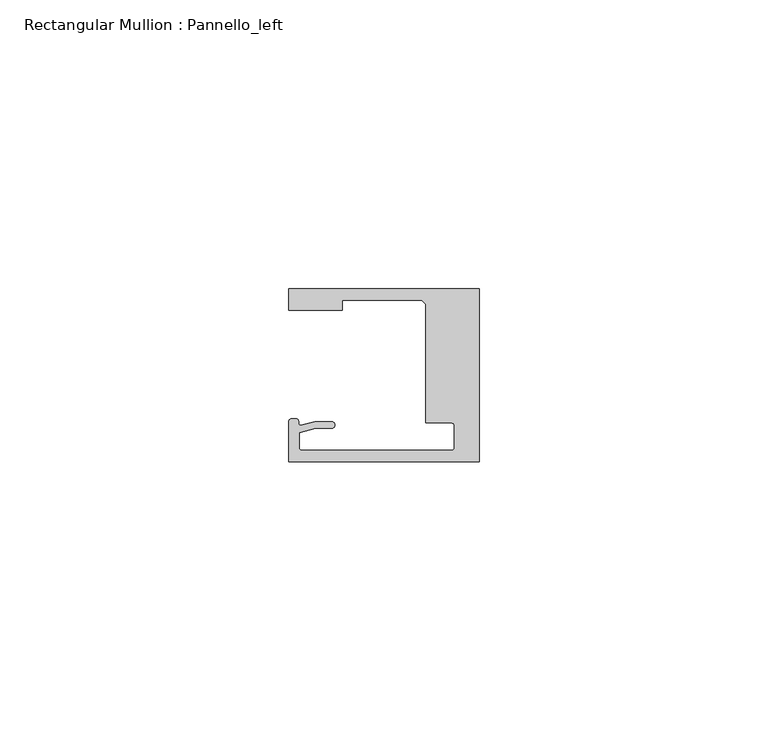
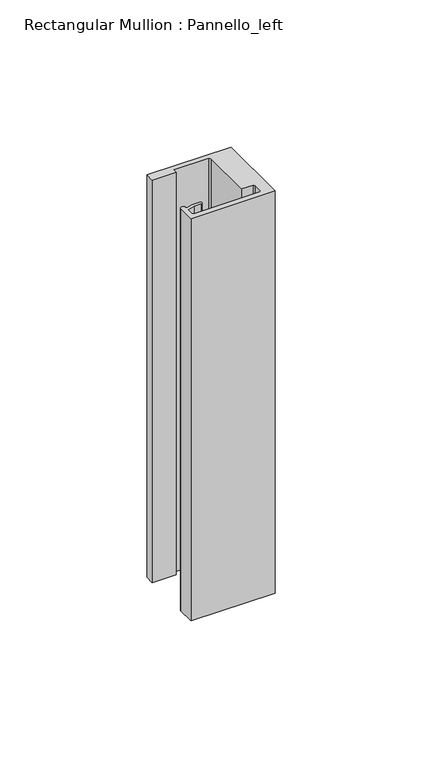
"""IFC4 building model written with IfcOpenShell, lengths in millimetres: member geometry, Rectangular Mullion : Pannello_left."""

import ifcopenshell
import ifcopenshell.guid

model = None  # the IFC model being written
_history = None  # IfcOwnerHistory: only IFC2X3 demands one
_inside = {}  # id of a spatial element -> (the spatial element, [elements in it])
_under = {}  # id of a project, library or spatial element -> (it, [spatial elements below it])
_declared = {}  # id of a project -> (the project, [libraries it declares])
_typed = {}  # id of a type object -> (the type object, [elements of that type])
_made_of = {}  # id of a material, layer set ... -> (it, [elements and type objects made of it])


def new_model(schema):
    """Start an empty IFC model of exactly this schema.

    Asked for "IFC4X3", IfcOpenShell would pick the latest addendum, in which some entities
    have other attributes; the version numbers below select the first issue.
    IFC2X3 requires an IfcOwnerHistory on every rooted entity: one is made here for all.
    """
    global model, _history
    if schema == "IFC4X3":
        model = ifcopenshell.file(schema_version=(4, 3, 0, 0))
    else:
        model = ifcopenshell.file(schema=schema)
    _inside.clear()
    _under.clear()
    _declared.clear()
    _typed.clear()
    _made_of.clear()
    _history = None
    if model.schema == "IFC2X3":
        org = make("IfcOrganization", Name="unknown")
        user = make(
            "IfcPersonAndOrganization",
            ThePerson=make("IfcPerson", FamilyName="unknown"),
            TheOrganization=org,
        )
        app = make(
            "IfcApplication",
            ApplicationDeveloper=org,
            Version="unknown",
            ApplicationFullName="unknown",
            ApplicationIdentifier="unknown",
        )
        _history = make(
            "IfcOwnerHistory",
            OwningUser=user,
            OwningApplication=app,
            ChangeAction="ADDED",
            CreationDate=0,
        )
    return model


def make(cls, **values):
    """One entity of the class cls with the attributes given. An attribute that is None is left unset."""
    return model.create_entity(
        cls, **{name: value for name, value in values.items() if value is not None}
    )


def rooted(cls, **values):
    """An entity with a GlobalId (a new one), such as an element, a storey or a relation."""
    return make(cls, GlobalId=ifcopenshell.guid.new(), OwnerHistory=_history, **values)


def si_unit(unit_type, name, prefix=None):
    """IfcSIUnit, for example si_unit("LENGTHUNIT", "METRE", prefix="MILLI")."""
    return make("IfcSIUnit", UnitType=unit_type, Prefix=prefix, Name=name)


def assignment(units):
    """IfcUnitAssignment: the units of a project."""
    return None if units is None else make("IfcUnitAssignment", Units=units)


def point(xyz):
    """IfcCartesianPoint."""
    return None if xyz is None else make("IfcCartesianPoint", Coordinates=xyz)


def direction(xyz):
    """IfcDirection."""
    return None if xyz is None else make("IfcDirection", DirectionRatios=xyz)


def frame(location, z_axis=None, x_axis=None):
    """IfcAxis2Placement3D, a coordinate frame: its origin and axes. An axis left out is left unset."""
    return make(
        "IfcAxis2Placement3D",
        Location=point(location),
        Axis=direction(z_axis),
        RefDirection=direction(x_axis),
    )


def origin():
    """The frame at (0, 0, 0) with its axes left unset."""
    return frame((0.0, 0.0, 0.0))


def place(relative_to, where):
    """IfcLocalPlacement: puts the frame where relative to a parent placement (None: the world)."""
    return make(
        "IfcLocalPlacement", PlacementRelTo=relative_to, RelativePlacement=where
    )


def context(
    kind, dimensions, precision=None, world=None, true_north=None, identifier=None
):
    """IfcGeometricRepresentationContext, for example the 3D "Model" context."""
    return make(
        "IfcGeometricRepresentationContext",
        ContextIdentifier=identifier,
        ContextType=kind,
        CoordinateSpaceDimension=dimensions,
        Precision=precision,
        WorldCoordinateSystem=world,
        TrueNorth=true_north,
    )


def project(units=None, contexts=None):
    """IfcProject with its units and contexts."""
    return rooted(
        "IfcProject",
        Name="project",
        RepresentationContexts=contexts,
        UnitsInContext=assignment(units),
    )


def spatial(cls, under=None, at=None, **own):
    """A site, building, storey or space (cls), placed at a placement, below another one or the project."""
    s = rooted(cls, ObjectPlacement=at, **own)
    if under is not None:
        _under.setdefault(under.id(), (under, []))[1].append(s)
    return s


def polyline(points):
    """IfcPolyline through the points."""
    return make("IfcPolyline", Points=[point(p) for p in points])


def circle_curve(where, radius):
    """IfcCircle in the frame where."""
    return make("IfcCircle", Position=where, Radius=radius)


def shape(context_of_items, identifier, shape_type, items):
    """IfcShapeRepresentation: the items that make up one representation, for example the "Body"."""
    return make(
        "IfcShapeRepresentation",
        ContextOfItems=context_of_items,
        RepresentationIdentifier=identifier,
        RepresentationType=shape_type,
        Items=items,
    )


def source(mapping_origin, context_of_items, identifier, shape_type, items):
    """IfcRepresentationMap: a shape defined once, which mapped items show again and again."""
    return make(
        "IfcRepresentationMap",
        MappingOrigin=mapping_origin,
        MappedRepresentation=shape(context_of_items, identifier, shape_type, items),
    )


def transform(
    local_origin,
    x_axis=None,
    y_axis=None,
    z_axis=None,
    scale=None,
    scale2=None,
    scale3=None,
    uniform=True,
):
    """IfcCartesianTransformationOperator3D, or its non-uniform kind. x_axis, y_axis, z_axis: its Axis1, 2, 3."""
    if uniform:
        return make(
            "IfcCartesianTransformationOperator3D",
            Axis1=direction(x_axis),
            Axis2=direction(y_axis),
            LocalOrigin=point(local_origin),
            Scale=scale,
            Axis3=direction(z_axis),
        )
    return make(
        "IfcCartesianTransformationOperator3DnonUniform",
        Axis1=direction(x_axis),
        Axis2=direction(y_axis),
        LocalOrigin=point(local_origin),
        Scale=scale,
        Axis3=direction(z_axis),
        Scale2=scale2,
        Scale3=scale3,
    )


def mapped(mapping_source, mapping_target):
    """IfcMappedItem: shows the shape of a source again, moved by a transform."""
    return make(
        "IfcMappedItem", MappingSource=mapping_source, MappingTarget=mapping_target
    )


def made_of(thing, what):
    """Note that an element or type object is made of a material, layer set ...; save() writes the relation."""
    if what is not None:
        _made_of.setdefault(what.id(), (what, []))[1].append(thing)
    return thing


def element(
    cls,
    number,
    at=None,
    inside=None,
    cuts=None,
    type_object=None,
    material=None,
    context=None,
    identifier="Body",
    shape_type=None,
    held_by="IfcProductDefinitionShape",
    body=None,
    shapes=None,
    **own,
):
    """One element of the class cls, such as IfcWall. Its Tag is "e" and its number.

    at: its placement. inside: the storey or other place that contains it. cuts: it is an
    opening in that element (IfcRelVoidsElement). A single representation is given by context,
    identifier, shape_type and body (its items); several are given by shapes. held_by: the class
    of the entity that holds the representations. save() writes the other relations.
    """
    e = rooted(cls, Tag="e%d" % number, ObjectPlacement=at, **own)
    if body is not None:
        shapes = [shape(context, identifier, shape_type, body)]
    if shapes is not None:
        e.Representation = make(held_by, Representations=shapes)
    if inside is not None:
        _inside.setdefault(inside.id(), (inside, []))[1].append(e)
    if cuts is not None:
        rooted(
            "IfcRelVoidsElement", RelatingBuildingElement=cuts, RelatedOpeningElement=e
        )
    if type_object is not None:
        _typed.setdefault(type_object.id(), (type_object, []))[1].append(e)
    return made_of(e, material)


def aggregate(whole, parts):
    """IfcRelAggregates: a whole, such as a stair, and the parts it consists of."""
    return rooted("IfcRelAggregates", RelatingObject=whole, RelatedObjects=parts)


def save(model, path):
    """Write the relations noted so far, then the file.

    IfcRelAggregates (storeys below a building ...), IfcRelContainedInSpatialStructure (elements
    in a storey), IfcRelDefinesByType, IfcRelAssociatesMaterial and IfcRelDeclares: one each for
    every whole, place, type object, material and project.
    """
    for whole, parts in _under.values():
        aggregate(whole, parts)
    for where, things in _inside.values():
        rooted(
            "IfcRelContainedInSpatialStructure",
            RelatedElements=things,
            RelatingStructure=where,
        )
    for kind, things in _typed.values():
        rooted("IfcRelDefinesByType", RelatedObjects=things, RelatingType=kind)
    for what, things in _made_of.values():
        rooted("IfcRelAssociatesMaterial", RelatedObjects=things, RelatingMaterial=what)
    for by, libraries in _declared.values():
        rooted("IfcRelDeclares", RelatingContext=by, RelatedDefinitions=libraries)
    model.write(path)


def plane_surface(at):
    """IfcPlane: the flat surface through the origin of the frame at, square to its z axis."""
    return make("IfcPlane", Position=at)


def cylinder_surface(at, radius):
    """IfcCylindricalSurface: all points at the distance radius from the z axis of the frame at."""
    return make("IfcCylindricalSurface", Position=at, Radius=radius)


def revolved_surface(curve, axis_point, axis_direction):
    """IfcSurfaceOfRevolution: the curve turned about the line through axis_point along axis_direction."""
    return make(
        "IfcSurfaceOfRevolution",
        SweptCurve=make("IfcArbitraryOpenProfileDef", ProfileType="CURVE", Curve=curve),
        AxisPosition=make("IfcAxis1Placement", Location=point(axis_point), Axis=direction(axis_direction)),
    )


def extruded_surface(curve, direction_of_extrusion, depth):
    """IfcSurfaceOfLinearExtrusion: the curve pushed along a direction by depth."""
    return make(
        "IfcSurfaceOfLinearExtrusion",
        SweptCurve=make("IfcArbitraryOpenProfileDef", ProfileType="CURVE", Curve=curve),
        ExtrudedDirection=direction(direction_of_extrusion),
        Depth=depth,
    )


def spline_curve(degree, points, multiplicities, knots, weights=None):
    """IfcBSplineCurveWithKnots; with weights, IfcRationalBSplineCurveWithKnots."""
    own = dict(
        Degree=degree,
        ControlPointsList=[point(p) for p in points],
        CurveForm="UNSPECIFIED",
        ClosedCurve=False,
        SelfIntersect=False,
        KnotMultiplicities=multiplicities,
        Knots=knots,
        KnotSpec="UNSPECIFIED",
    )
    if weights is None:
        return make("IfcBSplineCurveWithKnots", **own)
    return make("IfcRationalBSplineCurveWithKnots", WeightsData=weights, **own)


def advanced_brep(points, edges, surfaces, faces):
    """IfcAdvancedBrep: a solid bounded by faces that lie on surfaces and meet in shared edges.

    An edge is (start, end): straight between two places in points (the first is 0);
    or (start, end, curve); or (start, end, curve, False) where it runs against its curve.
    A face is (place in surfaces, loops), or (place, loops, False) where it looks against
    its surface's normal. A loop lists edges by number (the first is 1), with a minus sign
    where the edge is run from its end to its start. The first loop is the outer one.
    """
    corners = [point(p) for p in points]
    vertices = [make("IfcVertexPoint", VertexGeometry=c) for c in corners]
    made = []
    for start, end, *more in edges:
        made.append(
            make(
                "IfcEdgeCurve",
                EdgeStart=vertices[start],
                EdgeEnd=vertices[end],
                EdgeGeometry=more[0] if more else make("IfcPolyline", Points=[corners[start], corners[end]]),
                SameSense=more[1] if len(more) > 1 else True,
            )
        )
    hull = []
    for where, loops, *sense in faces:
        bounds = []
        for j, loop in enumerate(loops):
            ring = [make("IfcOrientedEdge", EdgeElement=made[abs(k) - 1], Orientation=k > 0) for k in loop]
            bounds.append(
                make(
                    "IfcFaceOuterBound" if j == 0 else "IfcFaceBound",
                    Bound=make("IfcEdgeLoop", EdgeList=ring),
                    Orientation=True,
                )
            )
        hull.append(make("IfcAdvancedFace", Bounds=bounds, FaceSurface=surfaces[where], SameSense=sense[0] if sense else True))
    return make("IfcAdvancedBrep", Outer=make("IfcClosedShell", CfsFaces=hull))


def rectangular_mullion_pannello_left_9b2e0e1e(model_context):
    return source(origin(), model_context, "Body", "AdvancedBrep", [
        advanced_brep(
        [(-33.0, 15.0, 0.0), (-33.0, 11.3000004, 0.0), (-23.700041, 11.3000004, 0.0), (-23.700041, 13.0000004, 0.0), (-10.0000103, 13.0000004, 0.0), (-9.2999726, 12.2999849, 0.0), (-9.2999726, -8.2500595, 0.0), (-4.7999726, -8.2500595, 0.0), (-4.2999726, -8.7500595, 0.0), (-4.2999726, -12.50001, 0.0), (-4.7999726, -13.00001, 0.0), (-30.69998, -13.00001, 0.0), (-31.19998, -12.50001, 0.0), (-31.19998, -9.9657591, 0.0), (-28.3419477, -9.1999523, 0.0), (-25.59998, -9.1999523, 0.0), (-25.59998, -7.9999523, 0.0), (-28.4999305, -7.9999523, 0.0), (-30.9223017, -8.6490241, 0.0), (-33.0000135, -8.0000472, 0.0), (-33.0000135, -15.0, 0.0), (0.0, -15.0, 0.0), (0.0, 15.0, 0.0), (-33.0, 15.0, -166.9999865), (0.0, 15.0, -166.9999865), (0.0, -15.0, -166.9999865), (-33.0000135, -15.0, -166.9999865), (-33.0000135, -8.0000472, -166.9999865), (-30.9223017, -8.6490241, -166.9999865), (-28.4999305, -7.9999523, -166.9999865), (-25.59998, -7.9999523, -166.9999865), (-25.59998, -9.1999523, -166.9999865), (-28.3419477, -9.1999523, -166.9999865), (-31.19998, -9.9657591, -166.9999865), (-31.19998, -12.50001, -166.9999865), (-30.69998, -13.00001, -166.9999865), (-4.7999726, -13.00001, -166.9999865), (-4.2999726, -12.50001, -166.9999865), (-4.2999726, -8.7500595, -166.9999865), (-4.7999726, -8.2500595, -166.9999865), (-9.2999726, -8.2500595, -166.9999865), (-9.2999726, 12.2999849, -166.9999865), (-10.0000103, 13.0000004, -166.9999865), (-23.700041, 13.0000004, -166.9999865), (-23.700041, 11.3000004, -166.9999865), (-33.0, 11.3000004, -166.9999865)],
        [
            (0, 1),
            (1, 2),
            (2, 3),
            (3, 4),
            (4, 5),
            (5, 6),
            (6, 7),
            (7, 8, circle_curve(frame((-4.7999726, -8.7500595, 0.0), z_axis=(0.0, 0.0, -1.0), x_axis=(0.0, 1.0, 0.0)), 0.5)),
            (8, 9),
            (9, 10, circle_curve(frame((-4.7999726, -12.50001, 0.0), z_axis=(0.0, 0.0, -1.0), x_axis=(1.0, 0.0, 0.0)), 0.5)),
            (10, 11),
            (11, 12, circle_curve(frame((-30.69998, -12.50001, 0.0), z_axis=(0.0, 0.0, -1.0), x_axis=(0.0, -1.0, 0.0)), 0.5)),
            (12, 13),
            (13, 14),
            (14, 15),
            (15, 16, circle_curve(frame((-25.59998, -8.5999523, 0.0), z_axis=(0.0, 0.0, 1.0), x_axis=(0.0, -1.0, 0.0)), 0.6)),
            (16, 17),
            (17, 18),
            (18, 19, spline_curve(3, [(-30.9223017, -8.6490241, 0.0), (-31.312054066, -8.717747958, 0.0), (-31.298563602, -8.366228555, 0.0), (-31.305645054, -7.690065204, 0.0), (-31.357433266, -7.563996614, 0.0), (-32.262327879, -7.456527435, 0.0), (-33.0000135, -7.457047519, 0.0), (-33.0000135, -8.0000472, 0.0)], [4, 2, 2, 4], [0.0, 0.001840817752199412, 0.004996616814974408, 0.007702013405570312])),
            (19, 20),
            (20, 21),
            (21, 22),
            (22, 0),
            (23, 24),
            (24, 25),
            (25, 26),
            (26, 27),
            (27, 28, spline_curve(3, [(-33.0000135, -8.0000472, -166.9999865), (-33.0000135, -7.457047519, -166.9999865), (-32.262327879, -7.456527435, -166.9999865), (-31.357433266, -7.563996614, -166.9999865), (-31.305645054, -7.690065204, -166.9999865), (-31.298563602, -8.366228555, -166.9999865), (-31.312054066, -8.717747958, -166.9999865), (-30.9223017, -8.6490241, -166.9999865)], [4, 2, 2, 4], [0.0, 0.0027053965905959043, 0.0058611956533709, 0.007702013405570312])),
            (28, 29),
            (29, 30),
            (30, 31, circle_curve(frame((-25.59998, -8.5999523, -166.9999865), z_axis=(0.0, 0.0, -1.0), x_axis=(0.0, -1.0, 0.0)), 0.6)),
            (31, 32),
            (32, 33),
            (33, 34),
            (34, 35, circle_curve(frame((-30.69998, -12.50001, -166.9999865), z_axis=(0.0, 0.0, 1.0), x_axis=(0.0, -1.0, 0.0)), 0.5)),
            (35, 36),
            (36, 37, circle_curve(frame((-4.7999726, -12.50001, -166.9999865), z_axis=(0.0, 0.0, 1.0), x_axis=(1.0, 0.0, 0.0)), 0.5)),
            (37, 38),
            (38, 39, circle_curve(frame((-4.7999726, -8.7500595, -166.9999865), z_axis=(0.0, 0.0, 1.0), x_axis=(0.0, 1.0, 0.0)), 0.5)),
            (39, 40),
            (40, 41),
            (41, 42),
            (42, 43),
            (43, 44),
            (44, 45),
            (45, 23),
            (0, 23),
            (45, 1),
            (44, 2),
            (43, 3),
            (42, 4),
            (41, 5),
            (40, 6),
            (39, 7),
            (38, 8),
            (37, 9),
            (36, 10),
            (35, 11),
            (34, 12),
            (33, 13),
            (32, 14),
            (31, 15),
            (30, 16),
            (29, 17),
            (28, 18),
            (27, 19),
            (26, 20),
            (25, 21),
            (24, 22),
        ],
        [
            plane_surface(frame((0.0, -36.2491502, 0.0), z_axis=(0.0, 0.0, 1.0), x_axis=(-1.0, 0.0, 0.0))),
            plane_surface(frame((0.0, -36.2491502, -166.9999865), z_axis=(0.0, 0.0, -1.0), x_axis=(-1.0, 0.0, 0.0))),
            plane_surface(frame((-33.0, 15.0, 0.0), z_axis=(-1.0, 0.0, 0.0), x_axis=(0.0, 0.0, -1.0))),
            plane_surface(frame((-33.0, 11.3000004, 0.0), z_axis=(0.0, -1.0, 0.0), x_axis=(0.0, 0.0, -1.0))),
            plane_surface(frame((-23.700041, 11.3000004, 0.0), z_axis=(1.0, 0.0, 0.0), x_axis=(0.0, 0.0, -1.0))),
            plane_surface(frame((-23.700041, 13.0000004, 0.0), z_axis=(0.0, -1.0, 0.0), x_axis=(0.0, 0.0, -1.0))),
            plane_surface(frame((-10.0000103, 13.0000004, 0.0), z_axis=(-0.7070955486277984, -0.7071180135668678, 0.0), x_axis=(0.0, 0.0, -1.0))),
            plane_surface(frame((-9.2999726, 12.2999849, 0.0), z_axis=(-1.0, 0.0, 0.0), x_axis=(0.0, 0.0, -1.0))),
            plane_surface(frame((-9.2999726, -8.2500595, 0.0), z_axis=(0.0, -1.0, 0.0), x_axis=(0.0, 0.0, -1.0))),
            revolved_surface(polyline([(-4.7999726, -8.2500595, -166.9999865), (-4.7999726, -8.2500595, 0.0)]), (-4.7999726, -8.7500595, 0.0), (0.0, 0.0, -1.0)),
            plane_surface(frame((-4.2999726, -8.7500595, 0.0), z_axis=(-1.0, 0.0, 0.0), x_axis=(0.0, 0.0, -1.0))),
            revolved_surface(polyline([(-4.2999726, -12.50001, -166.9999865), (-4.2999726, -12.50001, 0.0)]), (-4.7999726, -12.50001, 0.0), (0.0, 0.0, -1.0)),
            plane_surface(frame((-4.7999726, -13.00001, 0.0), z_axis=(0.0, 1.0, 0.0), x_axis=(0.0, 0.0, -1.0))),
            revolved_surface(polyline([(-30.69998, -13.00001, -166.9999865), (-30.69998, -13.00001, 0.0)]), (-30.69998, -12.50001, 0.0), (0.0, 0.0, -1.0)),
            plane_surface(frame((-31.19998, -12.50001, 0.0), z_axis=(1.0, 0.0, 0.0), x_axis=(0.0, 0.0, -1.0))),
            plane_surface(frame((-31.19998, -9.9657591, 0.0), z_axis=(0.25881883204288636, -0.9659258833782002, 0.0), x_axis=(0.0, 0.0, -1.0))),
            plane_surface(frame((-28.3419477, -9.1999523, 0.0), z_axis=(0.0, -1.0, 0.0), x_axis=(0.0, 0.0, -1.0))),
            cylinder_surface(frame((-25.59998, -8.5999523, 0.0), z_axis=(0.0, 0.0, 1.0), x_axis=(0.0, -1.0, 0.0)), 0.6),
            plane_surface(frame((-25.59998, -7.9999523, 0.0), z_axis=(0.0, 1.0, 0.0), x_axis=(0.0, 0.0, -1.0))),
            plane_surface(frame((-28.4999305, -7.9999523, 0.0), z_axis=(-0.25881883200192934, 0.9659258833891746, 0.0), x_axis=(0.0, 0.0, -1.0))),
            extruded_surface(spline_curve(3, [(-30.9223017, -8.6490241, -166.9999865), (-31.312054066, -8.717747958, -166.9999865), (-31.298563602, -8.366228555, -166.9999865), (-31.305645054, -7.690065204, -166.9999865), (-31.357433266, -7.563996614, -166.9999865), (-32.262327879, -7.456527435, -166.9999865), (-33.0000135, -7.457047519, -166.9999865), (-33.0000135, -8.0000472, -166.9999865)], [4, 2, 2, 4], [0.0, 0.001840817752199412, 0.004996616814974408, 0.007702013405570312]), (0.0, 0.0, 166.9999865), 166.9999865),
            plane_surface(frame((-33.0000135, -8.0000472, 0.0), z_axis=(-1.0, 0.0, 0.0), x_axis=(0.0, 0.0, -1.0))),
            plane_surface(frame((-33.0000135, -15.0, 0.0), z_axis=(0.0, -1.0, 0.0), x_axis=(0.0, 0.0, -1.0))),
            plane_surface(frame((0.0, -15.0, 0.0), z_axis=(1.0, 0.0, 0.0), x_axis=(0.0, 0.0, -1.0))),
            plane_surface(frame((0.0, 15.0, 0.0), z_axis=(0.0, 1.0, 0.0), x_axis=(0.0, 0.0, -1.0))),
        ],
        [
            (0, [[1, 2, 3, 4, 5, 6, 7, 8, 9, 10, 11, 12, 13, 14, 15, 16, 17, 18, 19, 20, 21, 22, 23]]),
            (1, [[24, 25, 26, 27, 28, 29, 30, 31, 32, 33, 34, 35, 36, 37, 38, 39, 40, 41, 42, 43, 44, 45, 46]]),
            (2, [[-1, 47, -46, 48]]),
            (3, [[-2, -48, -45, 49]]),
            (4, [[-3, -49, -44, 50]]),
            (5, [[-4, -50, -43, 51]]),
            (6, [[-5, -51, -42, 52]]),
            (7, [[-6, -52, -41, 53]]),
            (8, [[-7, -53, -40, 54]]),
            (9, [[-8, -54, -39, 55]]),
            (10, [[-9, -55, -38, 56]]),
            (11, [[-10, -56, -37, 57]]),
            (12, [[-11, -57, -36, 58]]),
            (13, [[-12, -58, -35, 59]]),
            (14, [[-13, -59, -34, 60]]),
            (15, [[-14, -60, -33, 61]]),
            (16, [[-15, -61, -32, 62]]),
            (17, [[-16, -62, -31, 63]]),
            (18, [[-17, -63, -30, 64]]),
            (19, [[-18, -64, -29, 65]]),
            (20, [[-19, -65, -28, 66]]),
            (21, [[-20, -66, -27, 67]]),
            (22, [[-21, -67, -26, 68]]),
            (23, [[-22, -68, -25, 69]]),
            (24, [[-23, -69, -24, -47]]),
        ],
    ),
    ])


if __name__ == "__main__":
    model = new_model("IFC4")
    model_context = context("Model", 3, world=origin())
    ifc_project = project(units=[si_unit("LENGTHUNIT", "METRE", prefix="MILLI")], contexts=[model_context])
    site = spatial("IfcSite", under=ifc_project)
    building = spatial("IfcBuilding", under=site)
    placement = place(None, origin())
    rectangular_mullion_pannello_left_shape = rectangular_mullion_pannello_left_9b2e0e1e(model_context)
    element("IfcMember", 1, ObjectType="Rectangular Mullion : Pannello_left", at=placement, inside=building, context=model_context, shape_type="MappedRepresentation", body=[
        mapped(rectangular_mullion_pannello_left_shape, transform((0.0, 0.0, 0.0), x_axis=(1.0, 0.0, 0.0), y_axis=(0.0, 1.0, 0.0), z_axis=(0.0, 0.0, 1.0))),
    ])
    save(model, "model.ifc")

# Revit data of these elements
# Type "Rectangular Mullion : Pannello_left"
#   built-in parameter 1007322 = 0.0984252 (stored number, unit not read)
#   built-in parameter 1007320 = 0.0305117 (stored number, unit not read)
